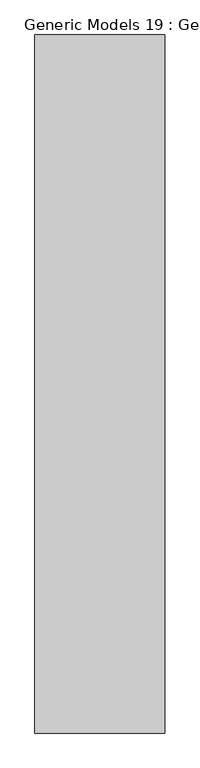
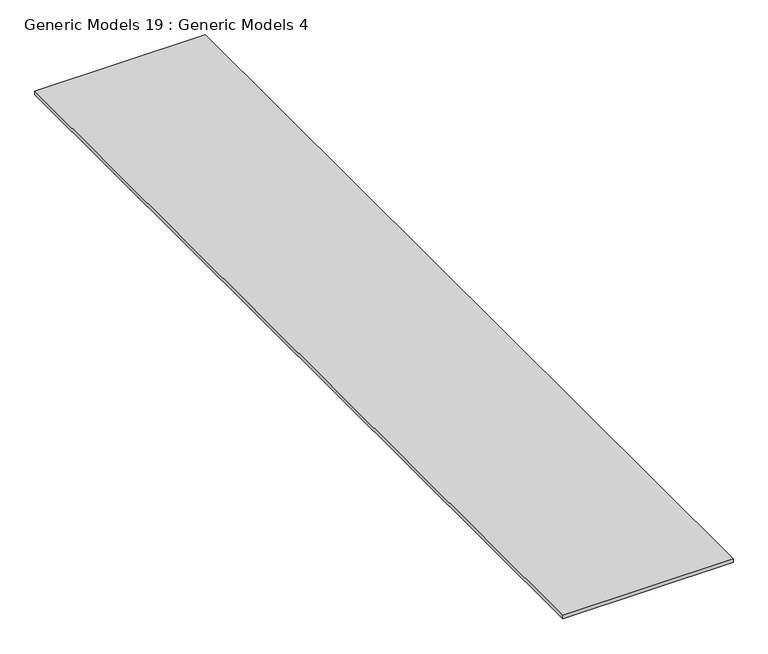
"""IFC4 building model written with IfcOpenShell, lengths in millimetres: proxy geometry, Generic Models 19 : Generic Models 4."""

from ifc_helpers import new_model, si_unit, frame, origin, place, context, project, spatial, polyline, outline, extrude, source, transform, mapped, element, save


def generic_models_19_generic_models_4_44e3a4d0(model_context):
    return source(origin(), model_context, "Body", "SweptSolid", [
        extrude(outline(polyline([(-8378.1251859, 7054.2769662), (-9257.8785997, 7054.2769662), (-9257.8785997, 11778.6769662), (-8378.1251859, 11778.6769662), (-8378.1251859, 7054.2769662)])), frame((0.0, 0.0, 126342.5425653), z_axis=(0.0, 0.0, 1.0), x_axis=(1.0, 0.0, 0.0)), (0.0, 0.0, 1.0), 19.05),
    ])


if __name__ == "__main__":
    model = new_model("IFC4")
    model_context = context("Model", 3, world=origin())
    ifc_project = project(units=[si_unit("LENGTHUNIT", "METRE", prefix="MILLI")], contexts=[model_context])
    site = spatial("IfcSite", under=ifc_project)
    building = spatial("IfcBuilding", under=site)
    placement = place(None, origin())
    generic_models_19_generic_models_4_shape = generic_models_19_generic_models_4_44e3a4d0(model_context)
    element("IfcBuildingElementProxy", 1, Name="Generic Models 19 : Generic Models 4", ObjectType="Generic Models 19 : Generic Models 4", at=placement, inside=building, context=model_context, shape_type="MappedRepresentation", body=[
        mapped(generic_models_19_generic_models_4_shape, transform((0.0, 0.0, 0.0), x_axis=(1.0, 0.0, 0.0), y_axis=(0.0, 1.0, 0.0), z_axis=(0.0, 0.0, 1.0))),
    ])
    save(model, "model.ifc")

# Revit data of these elements
# Element 1 (IfcBuildingElementProxy, "Generic Models 19 : Generic Models 4")
#   Materials on its faces: "_T&G FIRE RETARDANT WOOD SOFFIT O/ BUILDING PAPER"
# Materials
#   "_T&G FIRE RETARDANT WOOD SOFFIT O/ BUILDING PAPER": class "Generic", colour RGB 177 130 114, transparency 0, Cost = 0
